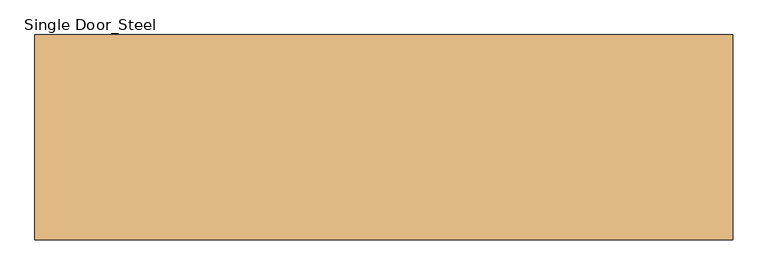
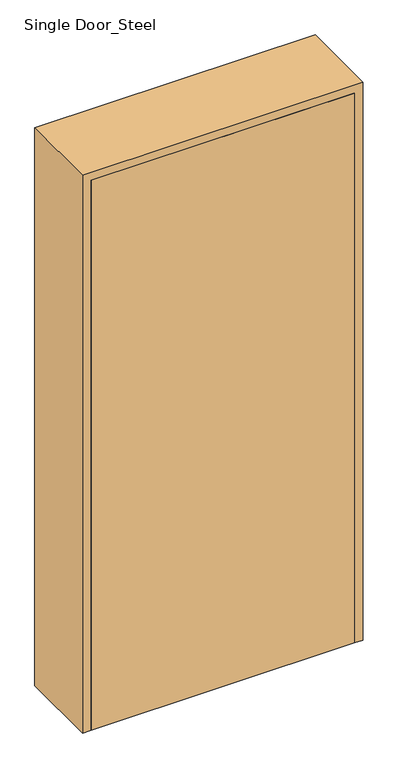
"""IFC4 building model written with IfcOpenShell, lengths in millimetres: door geometry, Single Door_Steel : H_DR_AMB_Single Door_Steel_W1000xH2100."""

from ifc_helpers import new_model, si_unit, origin, origin_with_axes, place, context, project, spatial, polyline, outline, extrude, faceted_brep, source, transform, mapped, element, save


def single_door_steel_29c29026(model_context):
    return source(origin(), model_context, "Body", "SolidModel", [
        extrude(outline(polyline([(470.0, -147.0), (-470.0, -147.0), (-470.0, -112.0), (470.0, -112.0), (470.0, -147.0)])), origin_with_axes(), (0.0, 0.0, 1.0), 2070.0),
        faceted_brep([(470.0, -147.0, 0.0), (470.0, -112.0, 0.0), (450.0, -112.0, 0.0), (450.0, 112.0, 0.0), (470.0, 112.0, 0.0), (470.0, 147.0, 0.0), (500.0, 147.0, 0.0), (500.0, -147.0, 0.0), (500.0, -147.0, 2100.0), (-500.0, -147.0, 2100.0), (-500.0, -147.0, 0.0), (-470.0, -147.0, 0.0), (-470.0, -147.0, 2070.0), (470.0, -147.0, 2070.0), (500.0, 147.0, 2100.0), (470.0, 147.0, 2070.0), (-470.0, 147.0, 2070.0), (-470.0, 147.0, 0.0), (-500.0, 147.0, 0.0), (-500.0, 147.0, 2100.0), (470.0, 112.0, 2070.0), (450.0, 112.0, 2050.0), (-450.0, 112.0, 2050.0), (-450.0, 112.0, 0.0), (-470.0, 112.0, 0.0), (-470.0, 112.0, 2070.0), (450.0, -112.0, 2050.0), (470.0, -112.0, 2070.0), (-470.0, -112.0, 2070.0), (-470.0, -112.0, 0.0), (-450.0, -112.0, 0.0), (-450.0, -112.0, 2050.0)], [[[0, 1, 2, 3, 4, 5, 6, 7]], [[7, 8, 9, 10, 11, 12, 13, 0]], [[6, 14, 8, 7]], [[5, 15, 16, 17, 18, 19, 14, 6]], [[4, 20, 15, 5]], [[3, 21, 22, 23, 24, 25, 20, 4]], [[2, 26, 21, 3]], [[1, 27, 28, 29, 30, 31, 26, 2]], [[0, 13, 27, 1]], [[12, 11, 29, 28]], [[11, 10, 18, 17, 24, 23, 30, 29]], [[19, 18, 10, 9]], [[25, 24, 17, 16]], [[31, 30, 23, 22]], [[14, 19, 9, 8]], [[20, 25, 16, 15]], [[26, 31, 22, 21]], [[13, 12, 28, 27]]]),
    ])


if __name__ == "__main__":
    model = new_model("IFC4")
    model_context = context("Model", 3, world=origin())
    ifc_project = project(units=[si_unit("LENGTHUNIT", "METRE", prefix="MILLI")], contexts=[model_context])
    site = spatial("IfcSite", under=ifc_project)
    building = spatial("IfcBuilding", under=site)
    placement = place(None, origin())
    single_door_steel_shape = single_door_steel_29c29026(model_context)
    element("IfcDoor", 1, ObjectType="Single Door_Steel : H_DR_AMB_Single Door_Steel_W1000xH2100", at=placement, inside=building, context=model_context, shape_type="MappedRepresentation", body=[
        mapped(single_door_steel_shape, transform((0.0, 0.0, 0.0), x_axis=(1.0, 0.0, 0.0), y_axis=(0.0, 1.0, 0.0), z_axis=(0.0, 0.0, 1.0))),
    ])
    save(model, "model.ifc")

# Revit data of these elements
# Type "Single Door_Steel : H_DR_AMB_Single Door_Steel_W1000xH2100"
#   Type Mark = "SD"
#   Analytic Construction = "<None>"
#   프레임 투영 외부. = 25 mm
#   프레임 투영 내부. = 25 mm
#   프레임 폭 = 75 mm
#   Height = 2100 mm
#   Width = 1000 mm
#   Define Thermal Properties by = 1
#   문 패널 = none
#   문 프레임 = none
#   Function = (empty or 0)
#   Wall Closure = (empty or 0)
